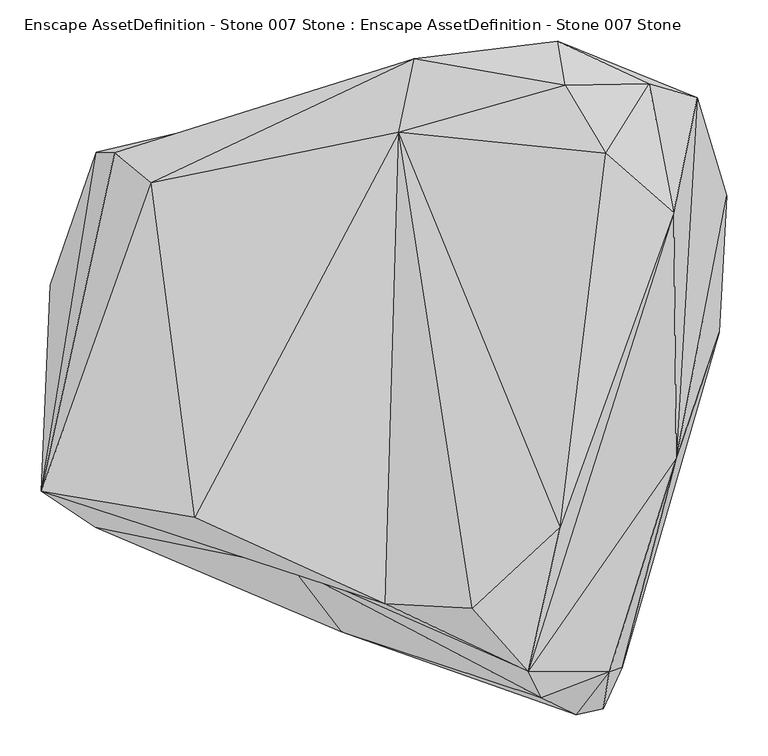
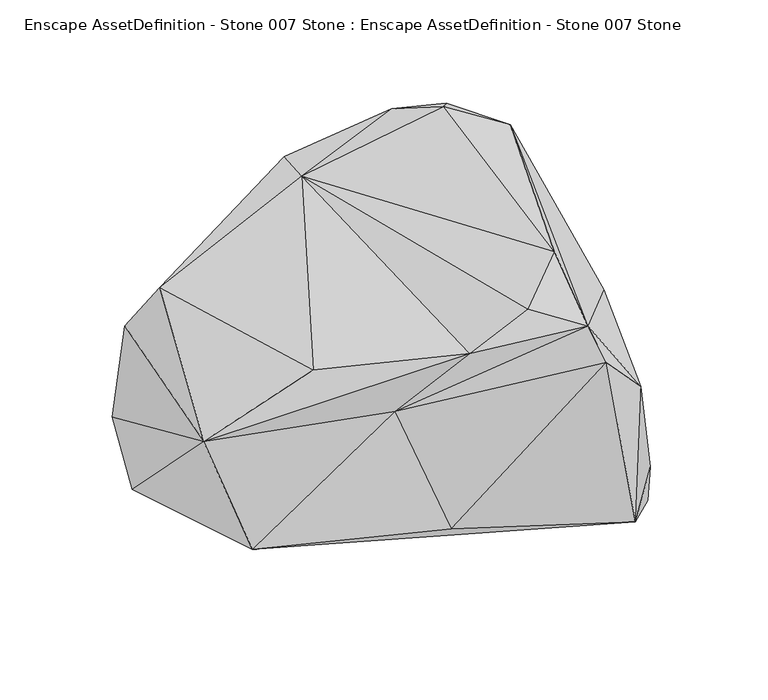
"""IFC4 building model written with IfcOpenShell, lengths in millimetres: geographic element geometry, Enscape AssetDefinition - Stone 007 Stone : Enscape AssetDefinition - Stone 007 Stone."""

from ifc_helpers import new_model, si_unit, origin, place, context, project, spatial, faceted_brep, source, transform, mapped, element, save


def enscape_assetdefinition_stone_007_stone_enscape_823d60b0(model_context):
    return source(origin(), model_context, "Body", "Brep", [
        faceted_brep([(224.847436, -174.5665222, 412.6452506), (363.1648719, 207.8361958, 383.7472498), (280.3442776, 280.4059386, 404.5871496), (333.5339725, 364.9718463, 341.812849), (391.9306397, 347.7776051, 246.3645637), (185.9779656, -350.0419855, 385.1563931), (366.1512434, -90.8051431, 237.0504588), (28.6185723, 305.9436381, 339.8826122), (230.8758497, 363.1937504, 367.601186), (117.9578826, -273.6137509, 396.4365423), (12.2159477, -268.3600187, 341.632843), (-272.9106843, 244.3567514, 261.6812289), (-219.8124826, -162.8050506, 326.1500895), (47.5888923, 395.4848349, 317.5778389), (221.7974216, 416.7802036, 318.7632561), (-317.4764216, 280.5779576, 179.1678965), (116.8490648, 389.3291354, 54.4019379), (-406.9549441, -131.0897321, 230.9613675), (-102.0385697, -223.5009223, 240.2436584), (-339.9760723, 281.7066908, 6.0771457), (-395.9980011, 119.5291281, -19.7330713), (-340.9456611, -174.9802381, 20.9592413), (249.5657355, 303.727001, -3.7451368), (418.8278019, 62.5018179, -46.8271337), (300.7983267, -345.4555273, -3.5024884), (244.4850355, -403.0079246, 8.300758), (-41.6648947, -301.9837141, 33.5023664), (284.8978937, -350.8773446, 231.6932976), (277.2813439, -395.7951069, 101.3454273), (427.9370606, 228.6422849, 6.5743756), (202.1468729, -382.6274574, 327.321589), (406.8664312, 288.1915569, 38.3036211)], [[[0, 1, 2]], [[1, 3, 2]], [[3, 1, 4]], [[0, 5, 1]], [[1, 6, 4]], [[5, 6, 1]], [[0, 2, 7]], [[7, 2, 8]], [[2, 3, 8]], [[0, 7, 9]], [[9, 5, 0]], [[9, 7, 10]], [[10, 5, 9]], [[11, 12, 7]], [[7, 12, 10]], [[7, 8, 13]], [[13, 11, 7]], [[8, 3, 14]], [[8, 14, 13]], [[15, 13, 16]], [[14, 16, 13]], [[13, 15, 11]], [[12, 11, 17]], [[11, 15, 17]], [[12, 17, 10]], [[17, 18, 10]], [[18, 5, 10]], [[15, 19, 17]], [[17, 20, 21]], [[18, 17, 21]], [[17, 19, 20]], [[19, 15, 16]], [[19, 22, 23]], [[20, 19, 23]], [[19, 16, 22]], [[23, 24, 20]], [[21, 20, 24]], [[21, 24, 25]], [[26, 18, 21]], [[26, 21, 25]], [[24, 6, 27]], [[23, 6, 24]], [[24, 27, 28]], [[24, 28, 25]], [[23, 29, 6]], [[22, 29, 23]], [[4, 6, 29]], [[27, 6, 5]], [[27, 30, 25]], [[5, 30, 27]], [[27, 25, 28]], [[25, 30, 26]], [[18, 26, 30]], [[5, 18, 30]], [[4, 31, 14]], [[3, 4, 14]], [[31, 4, 29]], [[31, 29, 22]], [[16, 14, 31]], [[16, 31, 22]]]),
    ])


if __name__ == "__main__":
    model = new_model("IFC4")
    model_context = context("Model", 3, world=origin())
    ifc_project = project(units=[si_unit("LENGTHUNIT", "METRE", prefix="MILLI")], contexts=[model_context])
    site = spatial("IfcSite", under=ifc_project)
    building = spatial("IfcBuilding", under=site)
    placement = place(None, origin())
    enscape_assetdefinition_stone_007_stone_enscape_shape = enscape_assetdefinition_stone_007_stone_enscape_823d60b0(model_context)
    element("IfcGeographicElement", 1, ObjectType="Enscape AssetDefinition - Stone 007 Stone : Enscape AssetDefinition - Stone 007 Stone", at=placement, inside=building, context=model_context, shape_type="MappedRepresentation", body=[
        mapped(enscape_assetdefinition_stone_007_stone_enscape_shape, transform((0.0, 0.0, 0.0), x_axis=(1.0, 0.0, 0.0), y_axis=(0.0, 1.0, 0.0), z_axis=(0.0, 0.0, 1.0))),
    ])
    save(model, "model.ifc")

# Revit data of these elements
# Type "Enscape AssetDefinition - Stone 007 Stone : Enscape AssetDefinition - Stone 007 Stone"
#   EnscapeAssetSource = "REMOTE"
#   EnscapeAssetId = "5933aa18-90c0-4cbc-9fcb-b684288696e0"
#   Height = 0.412645 m
#   EnscapeNativeAssetHeight = 0.412645 m
#   Default Elevation = 0
